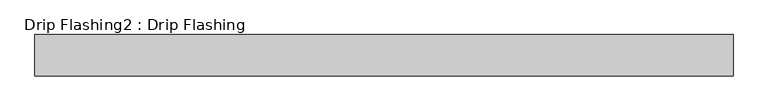
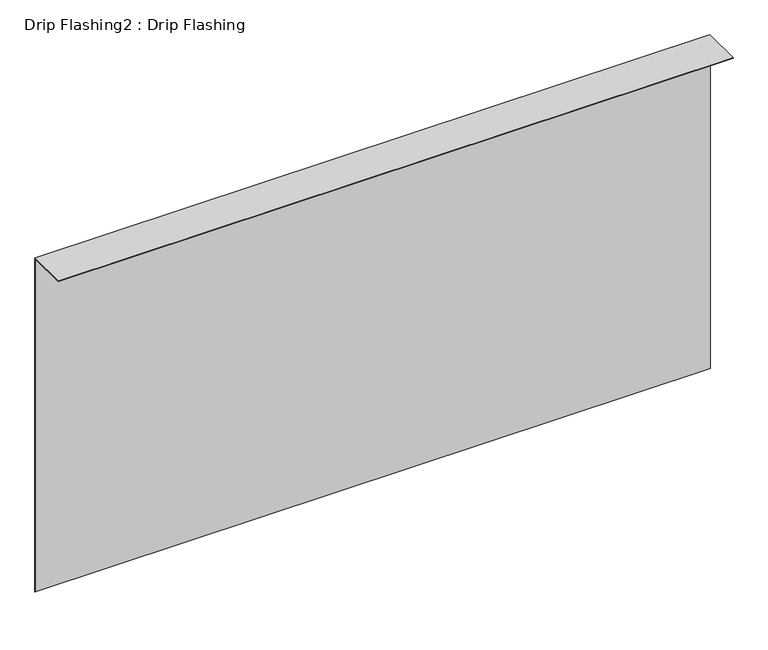
"""IFC4 building model written with IfcOpenShell, lengths in millimetres: proxy geometry, Drip Flashing2 : Drip Flashing."""

import ifcopenshell
import ifcopenshell.guid

model = None  # the IFC model being written
_history = None  # IfcOwnerHistory: only IFC2X3 demands one
_inside = {}  # id of a spatial element -> (the spatial element, [elements in it])
_under = {}  # id of a project, library or spatial element -> (it, [spatial elements below it])
_declared = {}  # id of a project -> (the project, [libraries it declares])
_typed = {}  # id of a type object -> (the type object, [elements of that type])
_made_of = {}  # id of a material, layer set ... -> (it, [elements and type objects made of it])


def new_model(schema):
    """Start an empty IFC model of exactly this schema.

    Asked for "IFC4X3", IfcOpenShell would pick the latest addendum, in which some entities
    have other attributes; the version numbers below select the first issue.
    IFC2X3 requires an IfcOwnerHistory on every rooted entity: one is made here for all.
    """
    global model, _history
    if schema == "IFC4X3":
        model = ifcopenshell.file(schema_version=(4, 3, 0, 0))
    else:
        model = ifcopenshell.file(schema=schema)
    _inside.clear()
    _under.clear()
    _declared.clear()
    _typed.clear()
    _made_of.clear()
    _history = None
    if model.schema == "IFC2X3":
        org = make("IfcOrganization", Name="unknown")
        user = make(
            "IfcPersonAndOrganization",
            ThePerson=make("IfcPerson", FamilyName="unknown"),
            TheOrganization=org,
        )
        app = make(
            "IfcApplication",
            ApplicationDeveloper=org,
            Version="unknown",
            ApplicationFullName="unknown",
            ApplicationIdentifier="unknown",
        )
        _history = make(
            "IfcOwnerHistory",
            OwningUser=user,
            OwningApplication=app,
            ChangeAction="ADDED",
            CreationDate=0,
        )
    return model


def make(cls, **values):
    """One entity of the class cls with the attributes given. An attribute that is None is left unset."""
    return model.create_entity(
        cls, **{name: value for name, value in values.items() if value is not None}
    )


def rooted(cls, **values):
    """An entity with a GlobalId (a new one), such as an element, a storey or a relation."""
    return make(cls, GlobalId=ifcopenshell.guid.new(), OwnerHistory=_history, **values)


def si_unit(unit_type, name, prefix=None):
    """IfcSIUnit, for example si_unit("LENGTHUNIT", "METRE", prefix="MILLI")."""
    return make("IfcSIUnit", UnitType=unit_type, Prefix=prefix, Name=name)


def assignment(units):
    """IfcUnitAssignment: the units of a project."""
    return None if units is None else make("IfcUnitAssignment", Units=units)


def point(xyz):
    """IfcCartesianPoint."""
    return None if xyz is None else make("IfcCartesianPoint", Coordinates=xyz)


def direction(xyz):
    """IfcDirection."""
    return None if xyz is None else make("IfcDirection", DirectionRatios=xyz)


def frame(location, z_axis=None, x_axis=None):
    """IfcAxis2Placement3D, a coordinate frame: its origin and axes. An axis left out is left unset."""
    return make(
        "IfcAxis2Placement3D",
        Location=point(location),
        Axis=direction(z_axis),
        RefDirection=direction(x_axis),
    )


def origin():
    """The frame at (0, 0, 0) with its axes left unset."""
    return frame((0.0, 0.0, 0.0))


def place(relative_to, where):
    """IfcLocalPlacement: puts the frame where relative to a parent placement (None: the world)."""
    return make(
        "IfcLocalPlacement", PlacementRelTo=relative_to, RelativePlacement=where
    )


def context(
    kind, dimensions, precision=None, world=None, true_north=None, identifier=None
):
    """IfcGeometricRepresentationContext, for example the 3D "Model" context."""
    return make(
        "IfcGeometricRepresentationContext",
        ContextIdentifier=identifier,
        ContextType=kind,
        CoordinateSpaceDimension=dimensions,
        Precision=precision,
        WorldCoordinateSystem=world,
        TrueNorth=true_north,
    )


def project(units=None, contexts=None):
    """IfcProject with its units and contexts."""
    return rooted(
        "IfcProject",
        Name="project",
        RepresentationContexts=contexts,
        UnitsInContext=assignment(units),
    )


def spatial(cls, under=None, at=None, **own):
    """A site, building, storey or space (cls), placed at a placement, below another one or the project."""
    s = rooted(cls, ObjectPlacement=at, **own)
    if under is not None:
        _under.setdefault(under.id(), (under, []))[1].append(s)
    return s


def polyline(points):
    """IfcPolyline through the points."""
    return make("IfcPolyline", Points=[point(p) for p in points])


def outline(outer, holes=None, kind="AREA"):
    """IfcArbitraryClosedProfileDef: a profile drawn as a closed curve; with holes, ...WithVoids."""
    if holes is None:
        return make("IfcArbitraryClosedProfileDef", ProfileType=kind, OuterCurve=outer)
    return make(
        "IfcArbitraryProfileDefWithVoids",
        ProfileType=kind,
        OuterCurve=outer,
        InnerCurves=holes,
    )


def extrude(swept, where, along, depth):
    """IfcExtrudedAreaSolid: the profile swept, set in the frame where, extruded along a direction by depth."""
    return make(
        "IfcExtrudedAreaSolid",
        SweptArea=swept,
        Position=where,
        ExtrudedDirection=direction(along),
        Depth=depth,
    )


def shape(context_of_items, identifier, shape_type, items):
    """IfcShapeRepresentation: the items that make up one representation, for example the "Body"."""
    return make(
        "IfcShapeRepresentation",
        ContextOfItems=context_of_items,
        RepresentationIdentifier=identifier,
        RepresentationType=shape_type,
        Items=items,
    )


def source(mapping_origin, context_of_items, identifier, shape_type, items):
    """IfcRepresentationMap: a shape defined once, which mapped items show again and again."""
    return make(
        "IfcRepresentationMap",
        MappingOrigin=mapping_origin,
        MappedRepresentation=shape(context_of_items, identifier, shape_type, items),
    )


def transform(
    local_origin,
    x_axis=None,
    y_axis=None,
    z_axis=None,
    scale=None,
    scale2=None,
    scale3=None,
    uniform=True,
):
    """IfcCartesianTransformationOperator3D, or its non-uniform kind. x_axis, y_axis, z_axis: its Axis1, 2, 3."""
    if uniform:
        return make(
            "IfcCartesianTransformationOperator3D",
            Axis1=direction(x_axis),
            Axis2=direction(y_axis),
            LocalOrigin=point(local_origin),
            Scale=scale,
            Axis3=direction(z_axis),
        )
    return make(
        "IfcCartesianTransformationOperator3DnonUniform",
        Axis1=direction(x_axis),
        Axis2=direction(y_axis),
        LocalOrigin=point(local_origin),
        Scale=scale,
        Axis3=direction(z_axis),
        Scale2=scale2,
        Scale3=scale3,
    )


def mapped(mapping_source, mapping_target):
    """IfcMappedItem: shows the shape of a source again, moved by a transform."""
    return make(
        "IfcMappedItem", MappingSource=mapping_source, MappingTarget=mapping_target
    )


def made_of(thing, what):
    """Note that an element or type object is made of a material, layer set ...; save() writes the relation."""
    if what is not None:
        _made_of.setdefault(what.id(), (what, []))[1].append(thing)
    return thing


def element(
    cls,
    number,
    at=None,
    inside=None,
    cuts=None,
    type_object=None,
    material=None,
    context=None,
    identifier="Body",
    shape_type=None,
    held_by="IfcProductDefinitionShape",
    body=None,
    shapes=None,
    **own,
):
    """One element of the class cls, such as IfcWall. Its Tag is "e" and its number.

    at: its placement. inside: the storey or other place that contains it. cuts: it is an
    opening in that element (IfcRelVoidsElement). A single representation is given by context,
    identifier, shape_type and body (its items); several are given by shapes. held_by: the class
    of the entity that holds the representations. save() writes the other relations.
    """
    e = rooted(cls, Tag="e%d" % number, ObjectPlacement=at, **own)
    if body is not None:
        shapes = [shape(context, identifier, shape_type, body)]
    if shapes is not None:
        e.Representation = make(held_by, Representations=shapes)
    if inside is not None:
        _inside.setdefault(inside.id(), (inside, []))[1].append(e)
    if cuts is not None:
        rooted(
            "IfcRelVoidsElement", RelatingBuildingElement=cuts, RelatedOpeningElement=e
        )
    if type_object is not None:
        _typed.setdefault(type_object.id(), (type_object, []))[1].append(e)
    return made_of(e, material)


def aggregate(whole, parts):
    """IfcRelAggregates: a whole, such as a stair, and the parts it consists of."""
    return rooted("IfcRelAggregates", RelatingObject=whole, RelatedObjects=parts)


def save(model, path):
    """Write the relations noted so far, then the file.

    IfcRelAggregates (storeys below a building ...), IfcRelContainedInSpatialStructure (elements
    in a storey), IfcRelDefinesByType, IfcRelAssociatesMaterial and IfcRelDeclares: one each for
    every whole, place, type object, material and project.
    """
    for whole, parts in _under.values():
        aggregate(whole, parts)
    for where, things in _inside.values():
        rooted(
            "IfcRelContainedInSpatialStructure",
            RelatedElements=things,
            RelatingStructure=where,
        )
    for kind, things in _typed.values():
        rooted("IfcRelDefinesByType", RelatedObjects=things, RelatingType=kind)
    for what, things in _made_of.values():
        rooted("IfcRelAssociatesMaterial", RelatedObjects=things, RelatingMaterial=what)
    for by, libraries in _declared.values():
        rooted("IfcRelDeclares", RelatingContext=by, RelatedDefinitions=libraries)
    model.write(path)


def drip_flashing2_drip_flashing_0b339f89(model_context):
    return source(origin(), model_context, "Body", "SweptSolid", [
        extrude(outline(polyline([(9742.7912647, 37600.3015275), (9625.4543522, 37600.3015275), (9625.4543522, 37601.8015275), (9744.2912647, 37601.8015275), (9744.2912647, 36556.696), (9742.7912647, 36556.696), (9742.7912647, 37600.3015275)])), frame((-9232.0719278, 0.0, 0.0), z_axis=(1.0, 0.0, 0.0), x_axis=(0.0, 1.0, 0.0)), (0.0, 0.0, 1.0), 1999.85),
    ])


if __name__ == "__main__":
    model = new_model("IFC4")
    model_context = context("Model", 3, world=origin())
    ifc_project = project(units=[si_unit("LENGTHUNIT", "METRE", prefix="MILLI")], contexts=[model_context])
    site = spatial("IfcSite", under=ifc_project)
    building = spatial("IfcBuilding", under=site)
    placement = place(None, origin())
    drip_flashing2_drip_flashing_shape = drip_flashing2_drip_flashing_0b339f89(model_context)
    element("IfcBuildingElementProxy", 1, Name="Drip Flashing2 : Drip Flashing", ObjectType="Drip Flashing2 : Drip Flashing", at=placement, inside=building, context=model_context, shape_type="MappedRepresentation", body=[
        mapped(drip_flashing2_drip_flashing_shape, transform((0.0, 0.0, 0.0), x_axis=(1.0, 0.0, 0.0), y_axis=(0.0, 1.0, 0.0), z_axis=(0.0, 0.0, 1.0))),
    ])
    save(model, "model.ifc")

# Revit data of these elements
# Type "Drip Flashing2 : Drip Flashing"
#   NameOverride = "Drip Flashing"
# Element 1 (IfcBuildingElementProxy, "Drip Flashing2 : Drip Flashing")
#   Materials on its faces: "(2) LAYERS OF ICE & WATER SHIELD (BITUTHANE) UNDER STUCCO"
# Materials
#   "(2) LAYERS OF ICE & WATER SHIELD (BITUTHANE) UNDER STUCCO": class "Unassigned", colour RGB 186 255 159, transparency 0, Cost = 0
